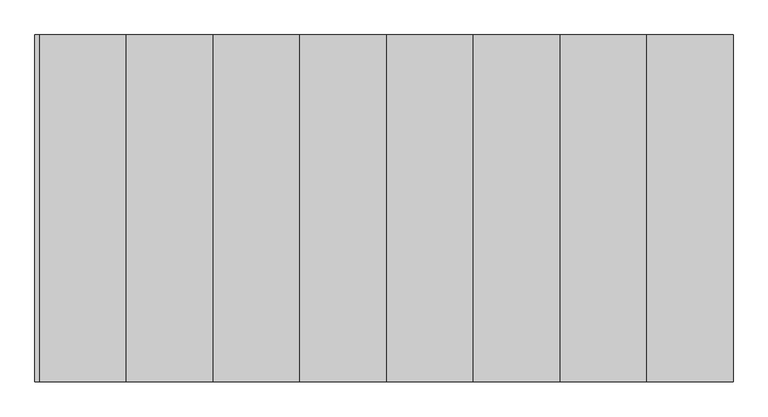
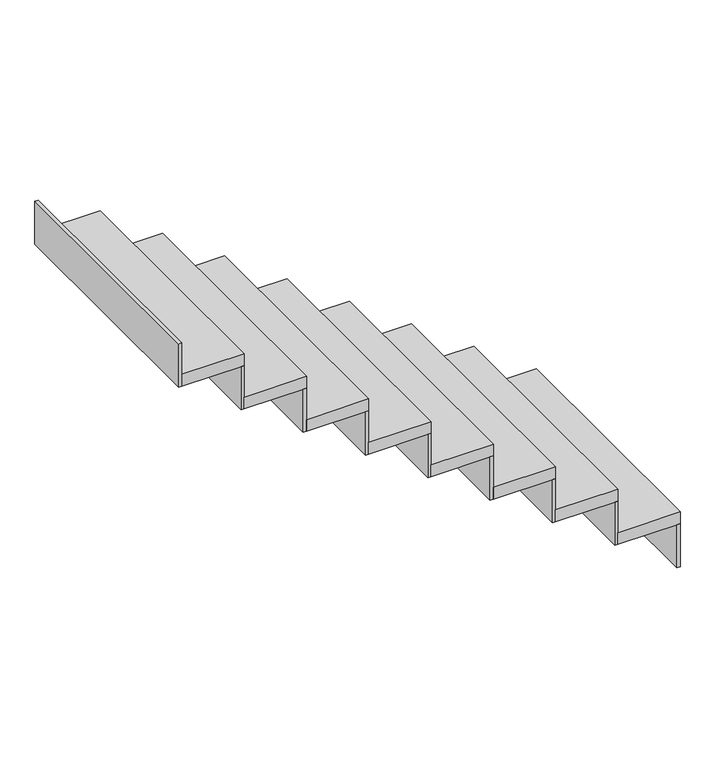
"""IFC4 building model written with IfcOpenShell, lengths in millimetres: stair flight geometry."""

from ifc_helpers import new_model, si_unit, frame, origin, place, context, project, spatial, polyline, outline, extrude, source, transform, mapped, element, save


def stair_flight_5f71a3ca(model_context):
    return source(origin(), model_context, "Body", "SweptSolid", [
        extrude(outline(polyline([(5264.0556606, 2510.81281), (5276.5556606, 2510.81281), (5276.5556606, 1510.81281), (5264.0556606, 1510.81281), (5264.0556606, 2510.81281)])), frame((0.0, 0.0, 1600.0), z_axis=(0.0, 0.0, 1.0), x_axis=(1.0, 0.0, 0.0)), (0.0, 0.0, 1.0), 183.3333333),
        extrude(outline(polyline([(5026.5556606, 1510.81281), (5026.5556606, 2510.81281), (5276.5556606, 2510.81281), (5276.5556606, 1510.81281), (5026.5556606, 1510.81281)])), frame((0.0, 0.0, 1783.3333333), z_axis=(0.0, 0.0, 1.0), x_axis=(1.0, 0.0, 0.0)), (0.0, 0.0, 1.0), 50.0),
        extrude(outline(polyline([(5014.0556606, 2510.81281), (5026.5556606, 2510.81281), (5026.5556606, 1510.81281), (5014.0556606, 1510.81281), (5014.0556606, 2510.81281)])), frame((0.0, 0.0, 1783.3333333), z_axis=(0.0, 0.0, 1.0), x_axis=(1.0, 0.0, 0.0)), (0.0, 0.0, 1.0), 183.3333333),
        extrude(outline(polyline([(4776.5556606, 1510.81281), (4776.5556606, 2510.81281), (5026.5556606, 2510.81281), (5026.5556606, 1510.81281), (4776.5556606, 1510.81281)])), frame((0.0, 0.0, 1966.6666667), z_axis=(0.0, 0.0, 1.0), x_axis=(1.0, 0.0, 0.0)), (0.0, 0.0, 1.0), 50.0),
        extrude(outline(polyline([(4764.0556606, 2510.81281), (4776.5556606, 2510.81281), (4776.5556606, 1510.81281), (4764.0556606, 1510.81281), (4764.0556606, 2510.81281)])), frame((0.0, 0.0, 1966.6666667), z_axis=(0.0, 0.0, 1.0), x_axis=(1.0, 0.0, 0.0)), (0.0, 0.0, 1.0), 183.3333333),
        extrude(outline(polyline([(4526.5556606, 1510.81281), (4526.5556606, 2510.81281), (4776.5556606, 2510.81281), (4776.5556606, 1510.81281), (4526.5556606, 1510.81281)])), frame((0.0, 0.0, 2150.0), z_axis=(0.0, 0.0, 1.0), x_axis=(1.0, 0.0, 0.0)), (0.0, 0.0, 1.0), 50.0),
        extrude(outline(polyline([(4514.0556606, 2510.81281), (4526.5556606, 2510.81281), (4526.5556606, 1510.81281), (4514.0556606, 1510.81281), (4514.0556606, 2510.81281)])), frame((0.0, 0.0, 2150.0), z_axis=(0.0, 0.0, 1.0), x_axis=(1.0, 0.0, 0.0)), (0.0, 0.0, 1.0), 183.3333333),
        extrude(outline(polyline([(4276.5556606, 1510.81281), (4276.5556606, 2510.81281), (4526.5556606, 2510.81281), (4526.5556606, 1510.81281), (4276.5556606, 1510.81281)])), frame((0.0, 0.0, 2333.3333333), z_axis=(0.0, 0.0, 1.0), x_axis=(1.0, 0.0, 0.0)), (0.0, 0.0, 1.0), 50.0),
        extrude(outline(polyline([(4264.0556606, 2510.81281), (4276.5556606, 2510.81281), (4276.5556606, 1510.81281), (4264.0556606, 1510.81281), (4264.0556606, 2510.81281)])), frame((0.0, 0.0, 2333.3333333), z_axis=(0.0, 0.0, 1.0), x_axis=(1.0, 0.0, 0.0)), (0.0, 0.0, 1.0), 183.3333333),
        extrude(outline(polyline([(4026.5556606, 1510.81281), (4026.5556606, 2510.81281), (4276.5556606, 2510.81281), (4276.5556606, 1510.81281), (4026.5556606, 1510.81281)])), frame((0.0, 0.0, 2516.6666667), z_axis=(0.0, 0.0, 1.0), x_axis=(1.0, 0.0, 0.0)), (0.0, 0.0, 1.0), 50.0),
        extrude(outline(polyline([(4014.0556606, 2510.81281), (4026.5556606, 2510.81281), (4026.5556606, 1510.81281), (4014.0556606, 1510.81281), (4014.0556606, 2510.81281)])), frame((0.0, 0.0, 2516.6666667), z_axis=(0.0, 0.0, 1.0), x_axis=(1.0, 0.0, 0.0)), (0.0, 0.0, 1.0), 183.3333333),
        extrude(outline(polyline([(3776.5556606, 1510.81281), (3776.5556606, 2510.81281), (4026.5556606, 2510.81281), (4026.5556606, 1510.81281), (3776.5556606, 1510.81281)])), frame((0.0, 0.0, 2700.0), z_axis=(0.0, 0.0, 1.0), x_axis=(1.0, 0.0, 0.0)), (0.0, 0.0, 1.0), 50.0),
        extrude(outline(polyline([(3764.0556606, 2510.81281), (3776.5556606, 2510.81281), (3776.5556606, 1510.81281), (3764.0556606, 1510.81281), (3764.0556606, 2510.81281)])), frame((0.0, 0.0, 2700.0), z_axis=(0.0, 0.0, 1.0), x_axis=(1.0, 0.0, 0.0)), (0.0, 0.0, 1.0), 183.3333333),
        extrude(outline(polyline([(3526.5556606, 1510.81281), (3526.5556606, 2510.81281), (3776.5556606, 2510.81281), (3776.5556606, 1510.81281), (3526.5556606, 1510.81281)])), frame((0.0, 0.0, 2883.3333333), z_axis=(0.0, 0.0, 1.0), x_axis=(1.0, 0.0, 0.0)), (0.0, 0.0, 1.0), 50.0),
        extrude(outline(polyline([(3514.0556606, 2510.81281), (3526.5556606, 2510.81281), (3526.5556606, 1510.81281), (3514.0556606, 1510.81281), (3514.0556606, 2510.81281)])), frame((0.0, 0.0, 2883.3333333), z_axis=(0.0, 0.0, 1.0), x_axis=(1.0, 0.0, 0.0)), (0.0, 0.0, 1.0), 183.3333333),
        extrude(outline(polyline([(3264.0556606, 2510.81281), (3276.5556606, 2510.81281), (3276.5556606, 1510.81281), (3264.0556606, 1510.81281), (3264.0556606, 2510.81281)])), frame((0.0, 0.0, 3066.6666667), z_axis=(0.0, 0.0, 1.0), x_axis=(1.0, 0.0, 0.0)), (0.0, 0.0, 1.0), 183.3333333),
        extrude(outline(polyline([(3276.5556606, 1510.81281), (3276.5556606, 2510.81281), (3526.5556606, 2510.81281), (3526.5556606, 1510.81281), (3276.5556606, 1510.81281)])), frame((0.0, 0.0, 3066.6666667), z_axis=(0.0, 0.0, 1.0), x_axis=(1.0, 0.0, 0.0)), (0.0, 0.0, 1.0), 50.0),
    ])


if __name__ == "__main__":
    model = new_model("IFC4")
    model_context = context("Model", 3, world=origin())
    ifc_project = project(units=[si_unit("LENGTHUNIT", "METRE", prefix="MILLI")], contexts=[model_context])
    site = spatial("IfcSite", under=ifc_project)
    building = spatial("IfcBuilding", under=site)
    placement = place(None, origin())
    stair_flight_shape = stair_flight_5f71a3ca(model_context)
    element("IfcStairFlight", 1, at=placement, inside=building, context=model_context, shape_type="MappedRepresentation", body=[
        mapped(stair_flight_shape, transform((0.0, 0.0, 0.0), x_axis=(1.0, 0.0, 0.0), y_axis=(0.0, 1.0, 0.0), z_axis=(0.0, 0.0, 1.0))),
    ])
    save(model, "model.ifc")
